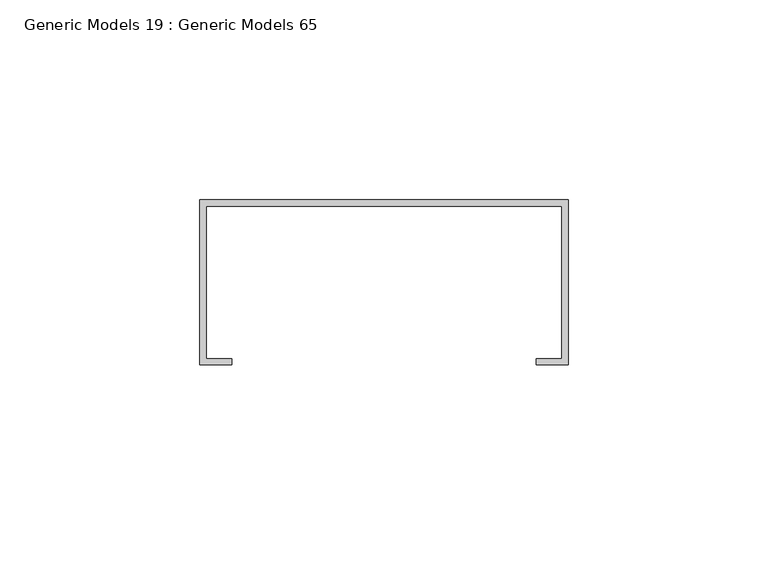
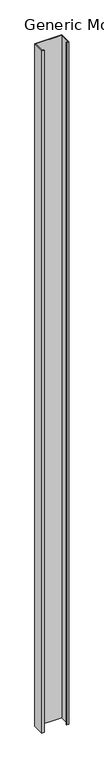
"""IFC4 building model written with IfcOpenShell, lengths in millimetres: proxy geometry, Generic Models 19 : Generic Models 65."""

from ifc_helpers import new_model, si_unit, frame, origin, place, context, project, spatial, polyline, outline, extrude, source, transform, mapped, element, save


def generic_models_19_generic_models_65_1c63a073(model_context):
    return source(origin(), model_context, "Body", "SweptSolid", [
        extrude(outline(polyline([(52558.3696108, 630.2375), (52650.4446108, 630.2375), (52650.4446108, 588.9625), (52642.5071108, 588.9625), (52642.5071108, 590.55), (52648.8571108, 590.55), (52648.8571108, 628.65), (52559.9571108, 628.65), (52559.9571108, 590.55), (52566.3071108, 590.55), (52566.3071108, 588.9625), (52558.3696108, 588.9625), (52558.3696108, 630.2375)])), frame((0.0, 0.0, -1922.8598206), z_axis=(0.0, 0.0, 1.0), x_axis=(1.0, 0.0, 0.0)), (0.0, 0.0, 1.0), 2454.275),
    ])


if __name__ == "__main__":
    model = new_model("IFC4")
    model_context = context("Model", 3, world=origin())
    ifc_project = project(units=[si_unit("LENGTHUNIT", "METRE", prefix="MILLI")], contexts=[model_context])
    site = spatial("IfcSite", under=ifc_project)
    building = spatial("IfcBuilding", under=site)
    placement = place(None, origin())
    generic_models_19_generic_models_65_shape = generic_models_19_generic_models_65_1c63a073(model_context)
    element("IfcBuildingElementProxy", 1, Name="Generic Models 19 : Generic Models 65", ObjectType="Generic Models 19 : Generic Models 65", at=placement, inside=building, context=model_context, shape_type="MappedRepresentation", body=[
        mapped(generic_models_19_generic_models_65_shape, transform((0.0, 0.0, 0.0), x_axis=(1.0, 0.0, 0.0), y_axis=(0.0, 1.0, 0.0), z_axis=(0.0, 0.0, 1.0))),
    ])
    save(model, "model.ifc")

# Revit data of these elements
# Element 1 (IfcBuildingElementProxy, "Generic Models 19 : Generic Models 65")
#   Materials on its faces: "METAL STUDS - SEE 'WALL TAG' & 'LAYER MATERIAL SCHEDULE' FOR GAUGE/SPACING & INSULATION TREATMENT, IF APPLICABLE"
# Materials
#   "METAL STUDS - SEE 'WALL TAG' & 'LAYER MATERIAL SCHEDULE' FOR GAUGE/SPACING & INSULATION TREATMENT, IF APPLICABLE": class "Unassigned", colour RGB 210 209 208, transparency 0, Keynote = "M05121300.02", Cost = 0
